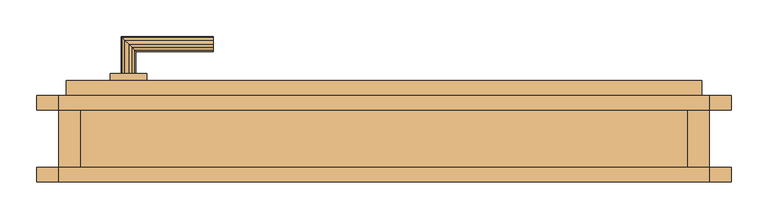
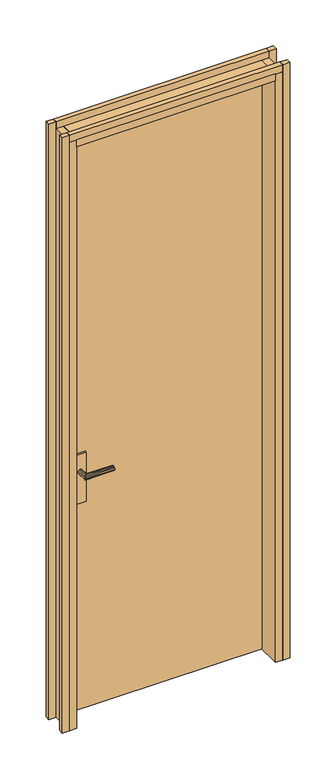
"""IFC4 building model written with IfcOpenShell, lengths in millimetres: door geometry, Tür."""

from ifc_helpers import new_model, si_unit, frame, origin, place, context, project, spatial, polyline, outline, extrude, faceted_brep, source, transform, mapped, element, save


def door_a8402586(model_context):
    return source(origin(), model_context, "Body", "SolidModel", [
        faceted_brep([(100.0, 128.0, 1198.660254), (95.0, 128.0, 1200.0), (90.0, 128.0, 1198.660254), (86.339746, 128.0, 1195.0), (85.0, 128.0, 1190.0), (86.339746, 128.0, 1185.0), (90.0, 128.0, 1181.339746), (95.0, 128.0, 1180.0), (100.0, 128.0, 1181.339746), (103.660254, 128.0, 1185.0), (105.0, 128.0, 1190.0), (103.660254, 128.0, 1195.0), (95.0, 168.0, 1200.0), (90.0, 173.0, 1198.660254), (86.339746, 176.660254, 1195.0), (85.0, 178.0, 1190.0), (86.339746, 176.660254, 1185.0), (90.0, 173.0, 1181.339746), (95.0, 168.0, 1180.0), (100.0, 163.0, 1181.339746), (103.660254, 159.339746, 1185.0), (105.0, 158.0, 1190.0), (103.660254, 159.339746, 1195.0), (100.0, 163.0, 1198.660254), (210.0, 173.0, 1198.660254), (210.0, 168.0, 1200.0), (210.0, 163.0, 1198.660254), (210.0, 159.339746, 1195.0), (210.0, 158.0, 1190.0), (210.0, 159.339746, 1185.0), (210.0, 163.0, 1181.339746), (210.0, 168.0, 1180.0), (210.0, 173.0, 1181.339746), (210.0, 176.660254, 1185.0), (210.0, 178.0, 1190.0), (210.0, 176.660254, 1195.0)], [[[0, 1, 2, 3, 4, 5, 6, 7, 8, 9, 10, 11]], [[2, 1, 12, 13]], [[3, 2, 13, 14]], [[4, 3, 14, 15]], [[5, 4, 15, 16]], [[6, 5, 16, 17]], [[7, 6, 17, 18]], [[8, 7, 18, 19]], [[9, 8, 19, 20]], [[10, 9, 20, 21]], [[11, 10, 21, 22]], [[0, 11, 22, 23]], [[1, 0, 23, 12]], [[24, 25, 26, 27, 28, 29, 30, 31, 32, 33, 34, 35]], [[13, 12, 25, 24]], [[14, 13, 24, 35]], [[15, 14, 35, 34]], [[16, 15, 34, 33]], [[17, 16, 33, 32]], [[18, 17, 32, 31]], [[19, 18, 31, 30]], [[20, 19, 30, 29]], [[21, 20, 29, 28]], [[22, 21, 28, 27]], [[23, 22, 27, 26]], [[12, 23, 26, 25]]]),
        extrude(outline(polyline([(875.0, 78.0), (10.0, 78.0), (10.0, 118.0), (875.0, 118.0), (875.0, 78.0)])), frame((0.0, 0.0, 140.0), z_axis=(0.0, 0.0, 1.0), x_axis=(1.0, 0.0, 0.0)), (0.0, 0.0, 1.0), 2570.0),
        extrude(outline(polyline([(885.0, 78.0), (0.0, 78.0), (0.0, 98.0), (885.0, 98.0), (885.0, 78.0)])), frame((0.0, 0.0, 2720.0), z_axis=(0.0, 0.0, 1.0), x_axis=(1.0, 0.0, 0.0)), (0.0, 0.0, 1.0), 30.0),
        extrude(outline(polyline([(120.0, 118.0), (70.0, 118.0), (70.0, 128.0), (120.0, 128.0), (120.0, 118.0)])), frame((0.0, 0.0, 1050.0), z_axis=(0.0, 0.0, 1.0), x_axis=(1.0, 0.0, 0.0)), (0.0, 0.0, 1.0), 215.0),
        extrude(outline(polyline([(855.0, -20.0), (30.0, -20.0), (30.0, 98.0), (855.0, 98.0), (855.0, -20.0)])), frame((0.0, 0.0, 2690.0), z_axis=(0.0, 0.0, 1.0), x_axis=(1.0, 0.0, 0.0)), (0.0, 0.0, 1.0), 30.0),
        extrude(outline(polyline([(885.0, -20.0), (0.0, -20.0), (0.0, 0.0), (885.0, 0.0), (885.0, -20.0)])), frame((0.0, 0.0, 2720.0), z_axis=(0.0, 0.0, 1.0), x_axis=(1.0, 0.0, 0.0)), (0.0, 0.0, 1.0), 30.0),
        extrude(outline(polyline([(70.0, 68.0), (70.0, 78.0), (120.0, 78.0), (120.0, 68.0), (70.0, 68.0)])), frame((0.0, 0.0, 1050.0), z_axis=(0.0, 0.0, 1.0), x_axis=(1.0, 0.0, 0.0)), (0.0, 0.0, 1.0), 215.0),
        extrude(outline(polyline([(0.0, 78.0), (-30.0, 78.0), (-30.0, 98.0), (0.0, 98.0), (0.0, 78.0)])), frame((0.0, 0.0, 140.0), z_axis=(0.0, 0.0, 1.0), x_axis=(1.0, 0.0, 0.0)), (0.0, 0.0, 1.0), 2610.0),
        extrude(outline(polyline([(915.0, 0.0), (915.0, -20.0), (885.0, -20.0), (885.0, 0.0), (915.0, 0.0)])), frame((0.0, 0.0, 140.0), z_axis=(0.0, 0.0, 1.0), x_axis=(1.0, 0.0, 0.0)), (0.0, 0.0, 1.0), 2610.0),
        extrude(outline(polyline([(30.0, -20.0), (0.0, -20.0), (0.0, 98.0), (30.0, 98.0), (30.0, -20.0)])), frame((0.0, 0.0, 140.0), z_axis=(0.0, 0.0, 1.0), x_axis=(1.0, 0.0, 0.0)), (0.0, 0.0, 1.0), 2580.0),
        extrude(outline(polyline([(885.0, -20.0), (855.0, -20.0), (855.0, 98.0), (885.0, 98.0), (885.0, -20.0)])), frame((0.0, 0.0, 140.0), z_axis=(0.0, 0.0, 1.0), x_axis=(1.0, 0.0, 0.0)), (0.0, 0.0, 1.0), 2580.0),
        extrude(outline(polyline([(915.0, 98.0), (915.0, 78.0), (885.0, 78.0), (885.0, 98.0), (915.0, 98.0)])), frame((0.0, 0.0, 140.0), z_axis=(0.0, 0.0, 1.0), x_axis=(1.0, 0.0, 0.0)), (0.0, 0.0, 1.0), 2610.0),
        faceted_brep([(90.0, 68.0, 1198.660254), (95.0, 68.0, 1200.0), (100.0, 68.0, 1198.660254), (103.660254, 68.0, 1195.0), (105.0, 68.0, 1190.0), (103.660254, 68.0, 1185.0), (100.0, 68.0, 1181.339746), (95.0, 68.0, 1180.0), (90.0, 68.0, 1181.339746), (86.339746, 68.0, 1185.0), (85.0, 68.0, 1190.0), (86.339746, 68.0, 1195.0), (95.0, 28.0, 1200.0), (90.0, 23.0, 1198.660254), (86.339746, 19.339746, 1195.0), (85.0, 18.0, 1190.0), (86.339746, 19.339746, 1185.0), (90.0, 23.0, 1181.339746), (95.0, 28.0, 1180.0), (100.0, 33.0, 1181.339746), (103.660254, 36.660254, 1185.0), (105.0, 38.0, 1190.0), (103.660254, 36.660254, 1195.0), (100.0, 33.0, 1198.660254), (210.0, 33.0, 1198.660254), (210.0, 28.0, 1200.0), (210.0, 23.0, 1198.660254), (210.0, 19.339746, 1195.0), (210.0, 18.0, 1190.0), (210.0, 19.339746, 1185.0), (210.0, 23.0, 1181.339746), (210.0, 28.0, 1180.0), (210.0, 33.0, 1181.339746), (210.0, 36.660254, 1185.0), (210.0, 38.0, 1190.0), (210.0, 36.660254, 1195.0)], [[[0, 1, 2, 3, 4, 5, 6, 7, 8, 9, 10, 11]], [[12, 1, 0, 13]], [[13, 0, 11, 14]], [[14, 11, 10, 15]], [[15, 10, 9, 16]], [[16, 9, 8, 17]], [[17, 8, 7, 18]], [[18, 7, 6, 19]], [[19, 6, 5, 20]], [[20, 5, 4, 21]], [[21, 4, 3, 22]], [[22, 3, 2, 23]], [[23, 2, 1, 12]], [[24, 25, 26, 27, 28, 29, 30, 31, 32, 33, 34, 35]], [[25, 12, 13, 26]], [[26, 13, 14, 27]], [[27, 14, 15, 28]], [[28, 15, 16, 29]], [[29, 16, 17, 30]], [[30, 17, 18, 31]], [[31, 18, 19, 32]], [[32, 19, 20, 33]], [[33, 20, 21, 34]], [[34, 21, 22, 35]], [[35, 22, 23, 24]], [[24, 23, 12, 25]]]),
        extrude(outline(polyline([(0.0, -20.0), (-30.0, -20.0), (-30.0, 0.0), (0.0, 0.0), (0.0, -20.0)])), frame((0.0, 0.0, 140.0), z_axis=(0.0, 0.0, 1.0), x_axis=(1.0, 0.0, 0.0)), (0.0, 0.0, 1.0), 2610.0),
    ])


if __name__ == "__main__":
    model = new_model("IFC4")
    model_context = context("Model", 3, world=origin())
    ifc_project = project(units=[si_unit("LENGTHUNIT", "METRE", prefix="MILLI")], contexts=[model_context])
    site = spatial("IfcSite", under=ifc_project)
    building = spatial("IfcBuilding", under=site)
    placement = place(None, origin())
    door_shape = door_a8402586(model_context)
    element("IfcDoor", 1, ObjectType="Tür", at=placement, inside=building, context=model_context, shape_type="MappedRepresentation", body=[
        mapped(door_shape, transform((0.0, 0.0, 0.0), x_axis=(1.0, 0.0, 0.0), y_axis=(0.0, 1.0, 0.0), z_axis=(0.0, 0.0, 1.0))),
    ])
    save(model, "model.ifc")

# Revit data of these elements
# Type "Tür"
#   Type Mark = "47"
# Element 1 (IfcDoor, "Tür")
#   Materials on its faces: "tuer_beschlag", "tuer_holzzarge"
# Materials
#   "tuer_beschlag": class "Unassigned", colour RGB 128 128 128, transparency 0
#   "tuer_holzzarge": class "Unassigned", colour RGB 255 255 255, transparency 0
